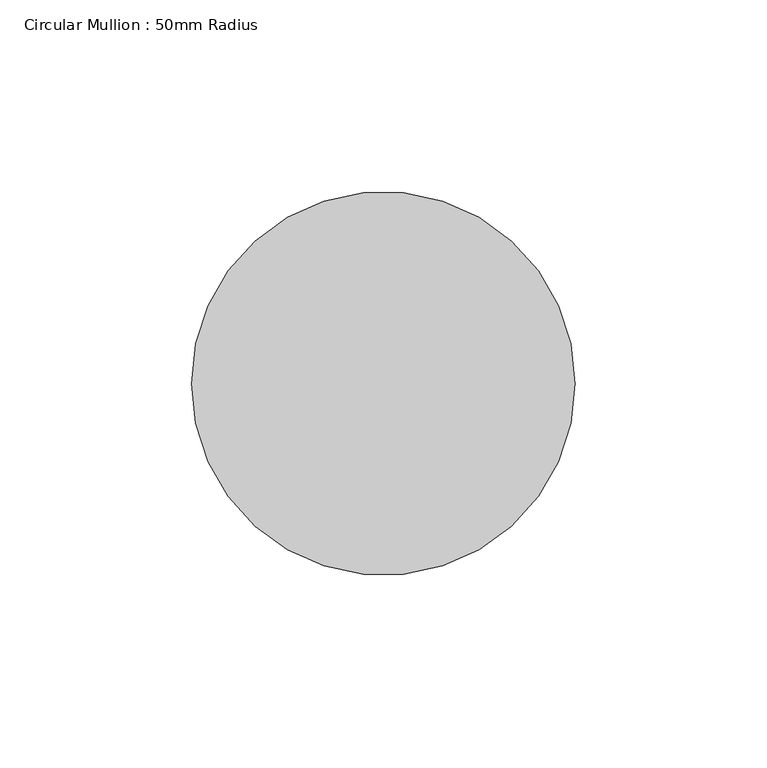
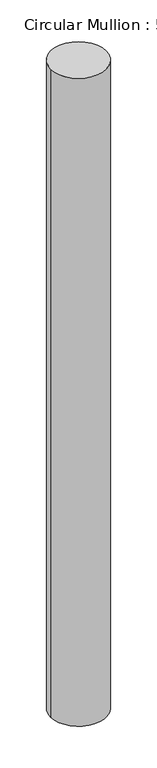
"""IFC4 building model written with IfcOpenShell, lengths in millimetres: member geometry, Circular Mullion : 50mm Radius."""

from ifc_helpers import new_model, si_unit, point, frame, origin, origin_2d, place, context, project, spatial, circle_curve, trimmed, segment, composite_curve, outline, extrude, source, transform, mapped, element, save


def circular_mullion_50mm_radius_b07aed92(model_context):
    return source(origin(), model_context, "Body", "SweptSolid", [
        extrude(outline(composite_curve([segment(trimmed(circle_curve(origin_2d(), 50.0), [point((50.0, 0.0))], [point((-50.0, 0.0))], False, "CARTESIAN"), True, "CONTINUOUS"), segment(trimmed(circle_curve(origin_2d(), 50.0), [point((-50.0, 0.0))], [point((50.0, 0.0))], False, "CARTESIAN"), True, "CONTINUOUS")], self_intersect=False)), frame((0.0, 0.0, -1233.4491472), z_axis=(0.0, 0.0, 1.0), x_axis=(1.0, 0.0, 0.0)), (0.0, 0.0, 1.0), 1233.4491472),
    ])


if __name__ == "__main__":
    model = new_model("IFC4")
    model_context = context("Model", 3, world=origin())
    ifc_project = project(units=[si_unit("LENGTHUNIT", "METRE", prefix="MILLI")], contexts=[model_context])
    site = spatial("IfcSite", under=ifc_project)
    building = spatial("IfcBuilding", under=site)
    placement = place(None, origin())
    circular_mullion_50mm_radius_shape = circular_mullion_50mm_radius_b07aed92(model_context)
    element("IfcMember", 1, ObjectType="Circular Mullion : 50mm Radius", at=placement, inside=building, context=model_context, shape_type="MappedRepresentation", body=[
        mapped(circular_mullion_50mm_radius_shape, transform((0.0, 0.0, 0.0), x_axis=(1.0, 0.0, 0.0), y_axis=(0.0, 1.0, 0.0), z_axis=(0.0, 0.0, 1.0))),
    ])
    save(model, "model.ifc")

# Revit data of these elements
# Type "Circular Mullion : 50mm Radius"
#   built-in parameter 1007350 = 0.164042 (stored number, unit not read)
# Element 1 (IfcMember, "Circular Mullion : 50mm Radius")
#   Materials on its faces: "Aluminium"
# Materials
#   "Aluminium": class "Metal", colour RGB 247 247 247, transparency 0, Description = "Aluminium 6061", Cost = 0
